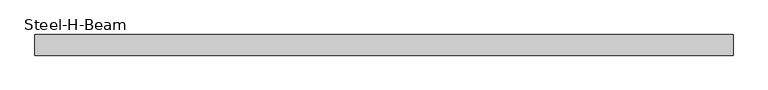
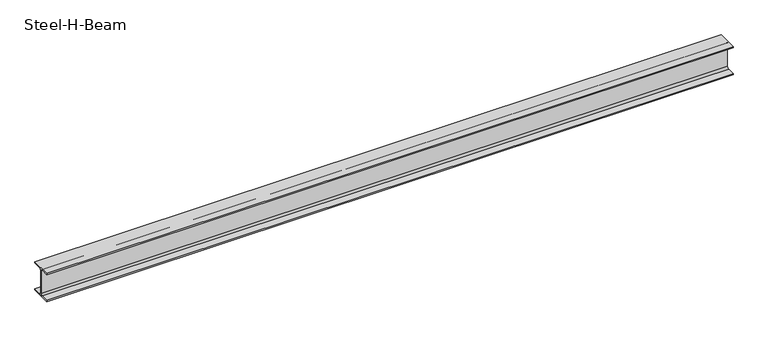
"""IFC4 building model written with IfcOpenShell, lengths in millimetres: beam geometry, Steel-H-Beam : BM121_H-294×200x8x12."""

from ifc_helpers import new_model, si_unit, point, frame, frame_2d, origin, place, context, project, spatial, polyline, circle_curve, trimmed, segment, composite_curve, outline, extrude, source, transform, mapped, element, save


def steel_h_beam_013c60b8(model_context):
    return source(origin(), model_context, "Body", "SweptSolid", [
        extrude(outline(composite_curve([segment(polyline([(100.0, -135.0), (100.0, -147.0), (-100.0, -147.0), (-100.0, -135.0), (-22.0, -135.0)]), True, "CONTINUOUS"), segment(trimmed(circle_curve(frame_2d((-22.0, -117.0)), 18.0), [point((-22.0, -135.0))], [point((-4.0, -117.0))], True, "CARTESIAN"), True, "CONTINUOUS"), segment(polyline([(-4.0, -117.0), (-4.0, 117.0)]), True, "CONTINUOUS"), segment(trimmed(circle_curve(frame_2d((-22.0, 117.0)), 18.0), [point((-4.0, 117.0))], [point((-22.0, 135.0))], True, "CARTESIAN"), True, "CONTINUOUS"), segment(polyline([(-22.0, 135.0), (-100.0, 135.0), (-100.0, 147.0), (100.0, 147.0), (100.0, 135.0), (22.0, 135.0)]), True, "CONTINUOUS"), segment(trimmed(circle_curve(frame_2d((22.0, 117.0)), 18.0), [point((22.0, 135.0))], [point((4.0, 117.0))], True, "CARTESIAN"), True, "CONTINUOUS"), segment(polyline([(4.0, 117.0), (4.0, -117.0)]), True, "CONTINUOUS"), segment(trimmed(circle_curve(frame_2d((22.0, -117.0)), 18.0), [point((4.0, -117.0))], [point((22.0, -135.0))], True, "CARTESIAN"), True, "CONTINUOUS"), segment(polyline([(22.0, -135.0), (100.0, -135.0)]), True, "CONTINUOUS")], self_intersect=False)), frame((-3380.0, 0.0, 0.0), z_axis=(1.0, 0.0, 0.0), x_axis=(0.0, 1.0, 0.0)), (0.0, 0.0, 1.0), 6760.0),
    ])


if __name__ == "__main__":
    model = new_model("IFC4")
    model_context = context("Model", 3, world=origin())
    ifc_project = project(units=[si_unit("LENGTHUNIT", "METRE", prefix="MILLI")], contexts=[model_context])
    site = spatial("IfcSite", under=ifc_project)
    building = spatial("IfcBuilding", under=site)
    placement = place(None, origin())
    steel_h_beam_shape = steel_h_beam_013c60b8(model_context)
    element("IfcBeam", 1, ObjectType="Steel-H-Beam : BM121_H-294×200x8x12", at=placement, inside=building, context=model_context, shape_type="MappedRepresentation", body=[
        mapped(steel_h_beam_shape, transform((0.0, 0.0, 0.0), x_axis=(1.0, 0.0, 0.0), y_axis=(0.0, 1.0, 0.0), z_axis=(0.0, 0.0, 1.0))),
    ])
    save(model, "model.ifc")

# Revit data of these elements
# Type "Steel-H-Beam : BM121_H-294×200x8x12"
#   Surface Area = 1.3411 m²/m
#   Section Area = 72.3812 cm²
#   Mass per Unit Length = 56.8193 kg/m
#   Length [instance default] = 3000 mm
#   B = 200 mm
#   H = 294 mm
#   r = 18 mm
#   tw = 8 mm
#   tf = 12 mm
#   hec_material4 [instance default] = none
#   hec_material3 [instance default] = none
#   hec_material2 [instance default] = none
#   hec_material1 [instance default] = none
#   Structural Material [instance default] = Steel, 45-345
#   Assembly Code = ""
# Element 1 (IfcBeam, "Steel-H-Beam : BM121_H-294×200x8x12")
#   hec_material3 = F01AC000-00002_Building/Shelter Fire Proofing Work_Intumescent Coating Type_1 hr. rating (UL 1709))
#   hec_material2 = S01AA010-00002_Main Steel Structure Fabrication Work_Shelter/Building_Steel Painting/Coating_for Fireproofed Steel Surface, Surface Preparation & Primer Coat
#   hec_material1 = S03AA028-00001_Main Steel Structure Erection Work_Shelter/Building_Medium Steel
#   Structural Material = S01AA002-00001_Main Steel Structure Fabrication Work_Shelter/Building_Medium Steel - Standard
#   Materials on its faces: "S01AA002-00001_Main Steel Structure Fabrication Work_Shelter/Building_Medium Steel - Standard"
# Materials
#   "Steel, 45-345": class "Metal", colour RGB 189 187 185, transparency 0, Description = "Steel 345 MPa", Cost = 0
#   "S01AA002-00001_Main Steel Structure Fabrication Work_Shelter/Building_Medium Steel - Standard": class "Metal", colour RGB 120 120 120, transparency 0, Comments = "(90KG/M>Weight≥30KG/M)", Description = "Structural steel 50ksi", W00) Work Master Code = "S01AA002-0001", W01) Work Master_Lv1 = "Main Steel Structure Fabrication Work", W02) Work Master_Lv2 = "Shelter/Building", W03) Work Master_Spec.1 = "Medium Steel - Standard (90KG/M>Weight≥30KG/M)", Cost = 0
#   "F01AC000-00002_Building/Shelter Fire Proofing Work_Intumescent Coating Type_1 hr. rating (UL 1709))": class "Metal", colour RGB 255 128 128, transparency 0, Description = "Paint finished steel", W00) Work Master Code = "F01AC000-00002", W01) Work Master_Lv1 = "Building/Shelter Fire Proofing Work", W02) Work Master_Lv2 = "Intumescent Coating Type", W03) Work Master_Spec.1 = "1 hr. rating (UL 1709)", Cost = 0
#   "S01AA010-00002_Main Steel Structure Fabrication Work_Shelter/Building_Steel Painting/Coating_for Fireproofed Steel Surface, Surface Preparation & Primer Coat": class "Metal", colour RGB 120 120 120, transparency 0, Description = "Paint finished steel", W00) Work Master Code = "SS01AA010-00002", W01) Work Master_Lv1 = "Main Steel Structure Fabrication Work", W02) Work Master_Lv2 = "Shelter/Building", W03) Work Master_Spec.1 = "Steel Painting/Coating", W04) Work Master_Spec.2 = "for Fireproofed Steel Surface, Surface Preparation & Primer Coat", Cost = 0
#   "S03AA028-00001_Main Steel Structure Erection Work_Shelter/Building_Medium Steel": class "Metal", colour RGB 120 120 120, transparency 0, Comments = "(90KG/M>Weight≥30KG/M)", Description = "Structural steel 50ksi", W00) Work Master Code = "S03AA028-0001", W01) Work Master_Lv1 = "Main Steel Structure Erection Work", W02) Work Master_Lv2 = "Shelter/Building", W03) Work Master_Spec.1 = "Medium Steel (90KG/M>Weight≥30KG/M)", Cost = 0
